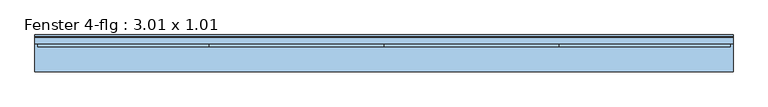
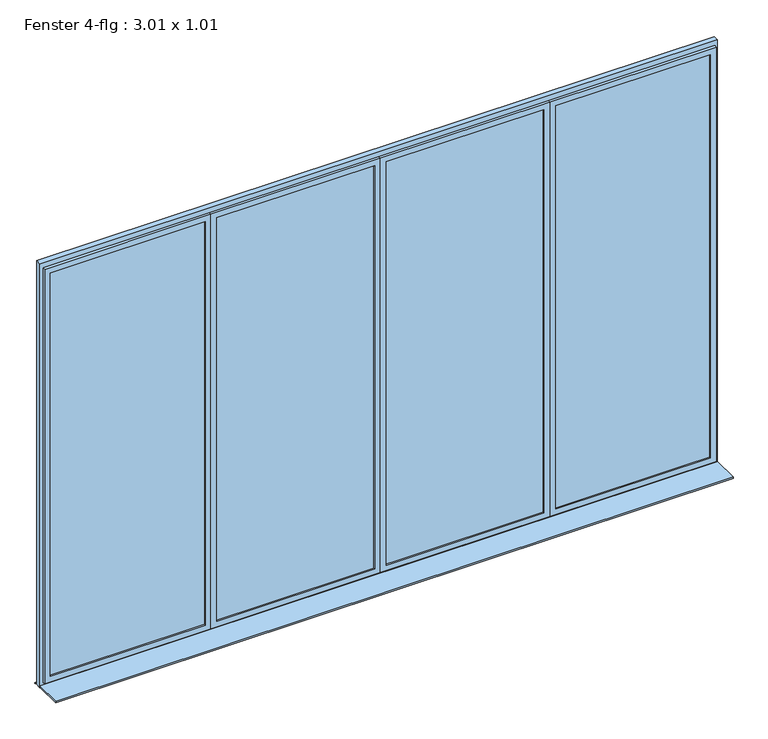
"""IFC4 building model written with IfcOpenShell, lengths in millimetres: window geometry, Fenster 4-flg : 3.01 x 1.01."""

import ifcopenshell
import ifcopenshell.guid

model = None  # the IFC model being written
_history = None  # IfcOwnerHistory: only IFC2X3 demands one
_inside = {}  # id of a spatial element -> (the spatial element, [elements in it])
_under = {}  # id of a project, library or spatial element -> (it, [spatial elements below it])
_declared = {}  # id of a project -> (the project, [libraries it declares])
_typed = {}  # id of a type object -> (the type object, [elements of that type])
_made_of = {}  # id of a material, layer set ... -> (it, [elements and type objects made of it])


def new_model(schema):
    """Start an empty IFC model of exactly this schema.

    Asked for "IFC4X3", IfcOpenShell would pick the latest addendum, in which some entities
    have other attributes; the version numbers below select the first issue.
    IFC2X3 requires an IfcOwnerHistory on every rooted entity: one is made here for all.
    """
    global model, _history
    if schema == "IFC4X3":
        model = ifcopenshell.file(schema_version=(4, 3, 0, 0))
    else:
        model = ifcopenshell.file(schema=schema)
    _inside.clear()
    _under.clear()
    _declared.clear()
    _typed.clear()
    _made_of.clear()
    _history = None
    if model.schema == "IFC2X3":
        org = make("IfcOrganization", Name="unknown")
        user = make(
            "IfcPersonAndOrganization",
            ThePerson=make("IfcPerson", FamilyName="unknown"),
            TheOrganization=org,
        )
        app = make(
            "IfcApplication",
            ApplicationDeveloper=org,
            Version="unknown",
            ApplicationFullName="unknown",
            ApplicationIdentifier="unknown",
        )
        _history = make(
            "IfcOwnerHistory",
            OwningUser=user,
            OwningApplication=app,
            ChangeAction="ADDED",
            CreationDate=0,
        )
    return model


def make(cls, **values):
    """One entity of the class cls with the attributes given. An attribute that is None is left unset."""
    return model.create_entity(
        cls, **{name: value for name, value in values.items() if value is not None}
    )


def rooted(cls, **values):
    """An entity with a GlobalId (a new one), such as an element, a storey or a relation."""
    return make(cls, GlobalId=ifcopenshell.guid.new(), OwnerHistory=_history, **values)


def si_unit(unit_type, name, prefix=None):
    """IfcSIUnit, for example si_unit("LENGTHUNIT", "METRE", prefix="MILLI")."""
    return make("IfcSIUnit", UnitType=unit_type, Prefix=prefix, Name=name)


def assignment(units):
    """IfcUnitAssignment: the units of a project."""
    return None if units is None else make("IfcUnitAssignment", Units=units)


def point(xyz):
    """IfcCartesianPoint."""
    return None if xyz is None else make("IfcCartesianPoint", Coordinates=xyz)


def direction(xyz):
    """IfcDirection."""
    return None if xyz is None else make("IfcDirection", DirectionRatios=xyz)


def frame(location, z_axis=None, x_axis=None):
    """IfcAxis2Placement3D, a coordinate frame: its origin and axes. An axis left out is left unset."""
    return make(
        "IfcAxis2Placement3D",
        Location=point(location),
        Axis=direction(z_axis),
        RefDirection=direction(x_axis),
    )


def origin():
    """The frame at (0, 0, 0) with its axes left unset."""
    return frame((0.0, 0.0, 0.0))


def place(relative_to, where):
    """IfcLocalPlacement: puts the frame where relative to a parent placement (None: the world)."""
    return make(
        "IfcLocalPlacement", PlacementRelTo=relative_to, RelativePlacement=where
    )


def context(
    kind, dimensions, precision=None, world=None, true_north=None, identifier=None
):
    """IfcGeometricRepresentationContext, for example the 3D "Model" context."""
    return make(
        "IfcGeometricRepresentationContext",
        ContextIdentifier=identifier,
        ContextType=kind,
        CoordinateSpaceDimension=dimensions,
        Precision=precision,
        WorldCoordinateSystem=world,
        TrueNorth=true_north,
    )


def project(units=None, contexts=None):
    """IfcProject with its units and contexts."""
    return rooted(
        "IfcProject",
        Name="project",
        RepresentationContexts=contexts,
        UnitsInContext=assignment(units),
    )


def spatial(cls, under=None, at=None, **own):
    """A site, building, storey or space (cls), placed at a placement, below another one or the project."""
    s = rooted(cls, ObjectPlacement=at, **own)
    if under is not None:
        _under.setdefault(under.id(), (under, []))[1].append(s)
    return s


def polyline(points):
    """IfcPolyline through the points."""
    return make("IfcPolyline", Points=[point(p) for p in points])


def outline(outer, holes=None, kind="AREA"):
    """IfcArbitraryClosedProfileDef: a profile drawn as a closed curve; with holes, ...WithVoids."""
    if holes is None:
        return make("IfcArbitraryClosedProfileDef", ProfileType=kind, OuterCurve=outer)
    return make(
        "IfcArbitraryProfileDefWithVoids",
        ProfileType=kind,
        OuterCurve=outer,
        InnerCurves=holes,
    )


def extrude(swept, where, along, depth):
    """IfcExtrudedAreaSolid: the profile swept, set in the frame where, extruded along a direction by depth."""
    return make(
        "IfcExtrudedAreaSolid",
        SweptArea=swept,
        Position=where,
        ExtrudedDirection=direction(along),
        Depth=depth,
    )


def faces_of(points, faces, orient=None, outer=None):
    """IfcFace entities. A face is a list of loops; a loop is a list of indices into points, from 0.

    orient and outer hold one flag for each loop. By default every Orientation is true, the
    first loop of a face is its IfcFaceOuterBound and the others are IfcFaceBound.
    """
    made = []
    for i, loops in enumerate(faces):
        bounds = []
        for j, loop in enumerate(loops):
            is_outer = j == 0 if outer is None else outer[i][j]
            bounds.append(
                make(
                    "IfcFaceOuterBound" if is_outer else "IfcFaceBound",
                    Bound=make("IfcPolyLoop", Polygon=[points[k] for k in loop]),
                    Orientation=True if orient is None else orient[i][j],
                )
            )
        made.append(make("IfcFace", Bounds=bounds))
    return made


def faceted_brep(points, faces, orient=None, outer=None, voids=None):
    """IfcFacetedBrep: a solid bounded by flat faces; with voids (closed shells), ...WithVoids."""
    shared = [point(p) for p in points]
    hull = make("IfcClosedShell", CfsFaces=faces_of(shared, faces, orient, outer))
    if voids is None:
        return make("IfcFacetedBrep", Outer=hull)
    return make(
        "IfcFacetedBrepWithVoids",
        Outer=hull,
        Voids=[
            make(cls, CfsFaces=faces_of(shared, fs, o, b)) for cls, fs, o, b in voids
        ],
    )


def shape(context_of_items, identifier, shape_type, items):
    """IfcShapeRepresentation: the items that make up one representation, for example the "Body"."""
    return make(
        "IfcShapeRepresentation",
        ContextOfItems=context_of_items,
        RepresentationIdentifier=identifier,
        RepresentationType=shape_type,
        Items=items,
    )


def source(mapping_origin, context_of_items, identifier, shape_type, items):
    """IfcRepresentationMap: a shape defined once, which mapped items show again and again."""
    return make(
        "IfcRepresentationMap",
        MappingOrigin=mapping_origin,
        MappedRepresentation=shape(context_of_items, identifier, shape_type, items),
    )


def transform(
    local_origin,
    x_axis=None,
    y_axis=None,
    z_axis=None,
    scale=None,
    scale2=None,
    scale3=None,
    uniform=True,
):
    """IfcCartesianTransformationOperator3D, or its non-uniform kind. x_axis, y_axis, z_axis: its Axis1, 2, 3."""
    if uniform:
        return make(
            "IfcCartesianTransformationOperator3D",
            Axis1=direction(x_axis),
            Axis2=direction(y_axis),
            LocalOrigin=point(local_origin),
            Scale=scale,
            Axis3=direction(z_axis),
        )
    return make(
        "IfcCartesianTransformationOperator3DnonUniform",
        Axis1=direction(x_axis),
        Axis2=direction(y_axis),
        LocalOrigin=point(local_origin),
        Scale=scale,
        Axis3=direction(z_axis),
        Scale2=scale2,
        Scale3=scale3,
    )


def mapped(mapping_source, mapping_target):
    """IfcMappedItem: shows the shape of a source again, moved by a transform."""
    return make(
        "IfcMappedItem", MappingSource=mapping_source, MappingTarget=mapping_target
    )


def made_of(thing, what):
    """Note that an element or type object is made of a material, layer set ...; save() writes the relation."""
    if what is not None:
        _made_of.setdefault(what.id(), (what, []))[1].append(thing)
    return thing


def element(
    cls,
    number,
    at=None,
    inside=None,
    cuts=None,
    type_object=None,
    material=None,
    context=None,
    identifier="Body",
    shape_type=None,
    held_by="IfcProductDefinitionShape",
    body=None,
    shapes=None,
    **own,
):
    """One element of the class cls, such as IfcWall. Its Tag is "e" and its number.

    at: its placement. inside: the storey or other place that contains it. cuts: it is an
    opening in that element (IfcRelVoidsElement). A single representation is given by context,
    identifier, shape_type and body (its items); several are given by shapes. held_by: the class
    of the entity that holds the representations. save() writes the other relations.
    """
    e = rooted(cls, Tag="e%d" % number, ObjectPlacement=at, **own)
    if body is not None:
        shapes = [shape(context, identifier, shape_type, body)]
    if shapes is not None:
        e.Representation = make(held_by, Representations=shapes)
    if inside is not None:
        _inside.setdefault(inside.id(), (inside, []))[1].append(e)
    if cuts is not None:
        rooted(
            "IfcRelVoidsElement", RelatingBuildingElement=cuts, RelatedOpeningElement=e
        )
    if type_object is not None:
        _typed.setdefault(type_object.id(), (type_object, []))[1].append(e)
    return made_of(e, material)


def aggregate(whole, parts):
    """IfcRelAggregates: a whole, such as a stair, and the parts it consists of."""
    return rooted("IfcRelAggregates", RelatingObject=whole, RelatedObjects=parts)


def save(model, path):
    """Write the relations noted so far, then the file.

    IfcRelAggregates (storeys below a building ...), IfcRelContainedInSpatialStructure (elements
    in a storey), IfcRelDefinesByType, IfcRelAssociatesMaterial and IfcRelDeclares: one each for
    every whole, place, type object, material and project.
    """
    for whole, parts in _under.values():
        aggregate(whole, parts)
    for where, things in _inside.values():
        rooted(
            "IfcRelContainedInSpatialStructure",
            RelatedElements=things,
            RelatingStructure=where,
        )
    for kind, things in _typed.values():
        rooted("IfcRelDefinesByType", RelatedObjects=things, RelatingType=kind)
    for what, things in _made_of.values():
        rooted("IfcRelAssociatesMaterial", RelatedObjects=things, RelatingMaterial=what)
    for by, libraries in _declared.values():
        rooted("IfcRelDeclares", RelatingContext=by, RelatedDefinitions=libraries)
    model.write(path)


def fenster_4_flg_3_01_x_1_01_20ed2dc3(model_context):
    return source(origin(), model_context, "Body", "SolidModel", [
        extrude(outline(polyline([(4150.75, 155.0), (4150.75, 95.0), (4090.75, 95.0), (4090.75, 155.0), (4150.75, 155.0)])), frame((0.0, 0.0, 1080.0), z_axis=(0.0, 0.0, 1.0), x_axis=(1.0, 0.0, 0.0)), (0.0, 0.0, 1.0), 4470.0),
        extrude(outline(polyline([(2400.5, 155.0), (2400.5, 95.0), (2340.5, 95.0), (2340.5, 155.0), (2400.5, 155.0)])), frame((0.0, 0.0, 1080.0), z_axis=(0.0, 0.0, 1.0), x_axis=(1.0, 0.0, 0.0)), (0.0, 0.0, 1.0), 4470.0),
        extrude(outline(polyline([(650.25, 155.0), (650.25, 95.0), (590.25, 95.0), (590.25, 155.0), (650.25, 155.0)])), frame((0.0, 0.0, 1080.0), z_axis=(0.0, 0.0, 1.0), x_axis=(1.0, 0.0, 0.0)), (0.0, 0.0, 1.0), 4470.0),
        extrude(outline(polyline([(5630.0, 5871.0), (5630.0, -1130.0), (1000.0, -1130.0), (1000.0, 5871.0), (5630.0, 5871.0)]), holes=[polyline([(5550.0, 5811.0), (1080.0, 5811.0), (1080.0, -1070.0), (5550.0, -1070.0), (5550.0, 5811.0)])]), frame((0.0, 95.0, 0.0), z_axis=(0.0, 1.0, 0.0), x_axis=(0.0, 0.0, 1.0)), (0.0, 0.0, 1.0), 60.0),
        faceted_brep([(4120.75, 95.0, 5580.0), (4120.75, 65.0, 5580.0), (4120.75, 65.0, 1050.0), (4120.75, 95.0, 1050.0), (2370.5, 65.0, 5580.0), (2370.5, 65.0, 1050.0), (4060.75, 65.0, 1110.0), (2430.5, 65.0, 1110.0), (2430.5, 65.0, 5520.0), (4060.75, 65.0, 5520.0), (2370.5, 95.0, 1050.0), (2370.5, 95.0, 5580.0), (4090.75, 95.0, 5550.0), (2400.5, 95.0, 5550.0), (2400.5, 95.0, 1080.0), (4090.75, 95.0, 1080.0), (4090.75, 125.0, 5550.0), (4090.75, 125.0, 1080.0), (2400.5, 125.0, 1080.0), (2400.5, 125.0, 5550.0), (4060.75, 125.0, 5520.0), (2430.5, 125.0, 5520.0), (2430.5, 125.0, 1110.0), (4060.75, 125.0, 1110.0)], [[[0, 1, 2, 3]], [[1, 4, 5, 2], [6, 7, 8, 9]], [[3, 2, 5, 10]], [[3, 10, 11, 0], [12, 13, 14, 15]], [[16, 12, 15, 17]], [[17, 15, 14, 18]], [[17, 18, 19, 16], [20, 21, 22, 23]], [[9, 20, 23, 6]], [[6, 23, 22, 7]], [[10, 5, 4, 11]], [[18, 14, 13, 19]], [[7, 22, 21, 8]], [[11, 4, 1, 0]], [[19, 13, 12, 16]], [[8, 21, 20, 9]]]),
        faceted_brep([(2370.5, 95.0, 5580.0), (2370.5, 65.0, 5580.0), (2370.5, 65.0, 1050.0), (2370.5, 95.0, 1050.0), (620.25, 65.0, 5580.0), (620.25, 65.0, 1050.0), (2310.5, 65.0, 1110.0), (680.25, 65.0, 1110.0), (680.25, 65.0, 5520.0), (2310.5, 65.0, 5520.0), (620.25, 95.0, 1050.0), (620.25, 95.0, 5580.0), (2340.5, 95.0, 5550.0), (650.25, 95.0, 5550.0), (650.25, 95.0, 1080.0), (2340.5, 95.0, 1080.0), (2340.5, 125.0, 5550.0), (2340.5, 125.0, 1080.0), (650.25, 125.0, 1080.0), (650.25, 125.0, 5550.0), (2310.5, 125.0, 5520.0), (680.25, 125.0, 5520.0), (680.25, 125.0, 1110.0), (2310.5, 125.0, 1110.0)], [[[0, 1, 2, 3]], [[1, 4, 5, 2], [6, 7, 8, 9]], [[3, 2, 5, 10]], [[3, 10, 11, 0], [12, 13, 14, 15]], [[16, 12, 15, 17]], [[17, 15, 14, 18]], [[17, 18, 19, 16], [20, 21, 22, 23]], [[9, 20, 23, 6]], [[6, 23, 22, 7]], [[10, 5, 4, 11]], [[18, 14, 13, 19]], [[7, 22, 21, 8]], [[11, 4, 1, 0]], [[19, 13, 12, 16]], [[8, 21, 20, 9]]]),
        faceted_brep([(620.25, 95.0, 5580.0), (620.25, 65.0, 5580.0), (620.25, 65.0, 1050.0), (620.25, 95.0, 1050.0), (-1100.0, 65.0, 5580.0), (-1100.0, 65.0, 1050.0), (560.25, 65.0, 1110.0), (-1040.0, 65.0, 1110.0), (-1040.0, 65.0, 5520.0), (560.25, 65.0, 5520.0), (-1100.0, 95.0, 1050.0), (-1100.0, 95.0, 5580.0), (590.25, 95.0, 5550.0), (-1070.0, 95.0, 5550.0), (-1070.0, 95.0, 1080.0), (590.25, 95.0, 1080.0), (590.25, 125.0, 5550.0), (590.25, 125.0, 1080.0), (-1070.0, 125.0, 1080.0), (-1070.0, 125.0, 5550.0), (560.25, 125.0, 5520.0), (-1040.0, 125.0, 5520.0), (-1040.0, 125.0, 1110.0), (560.25, 125.0, 1110.0)], [[[0, 1, 2, 3]], [[1, 4, 5, 2], [6, 7, 8, 9]], [[3, 2, 5, 10]], [[3, 10, 11, 0], [12, 13, 14, 15]], [[16, 12, 15, 17]], [[17, 15, 14, 18]], [[17, 18, 19, 16], [20, 21, 22, 23]], [[9, 20, 23, 6]], [[6, 23, 22, 7]], [[10, 5, 4, 11]], [[18, 14, 13, 19]], [[7, 22, 21, 8]], [[11, 4, 1, 0]], [[19, 13, 12, 16]], [[8, 21, 20, 9]]]),
        faceted_brep([(5841.0, 95.0, 5580.0), (5841.0, 65.0, 5580.0), (5841.0, 65.0, 1050.0), (5841.0, 95.0, 1050.0), (4120.75, 65.0, 5580.0), (4120.75, 65.0, 1050.0), (5781.0, 65.0, 1110.0), (4180.75, 65.0, 1110.0), (4180.75, 65.0, 5520.0), (5781.0, 65.0, 5520.0), (4120.75, 95.0, 1050.0), (4120.75, 95.0, 5580.0), (5811.0, 95.0, 5550.0), (4150.75, 95.0, 5550.0), (4150.75, 95.0, 1080.0), (5811.0, 95.0, 1080.0), (5811.0, 125.0, 5550.0), (5811.0, 125.0, 1080.0), (4150.75, 125.0, 1080.0), (4150.75, 125.0, 5550.0), (5781.0, 125.0, 5520.0), (4180.75, 125.0, 5520.0), (4180.75, 125.0, 1110.0), (5781.0, 125.0, 1110.0)], [[[0, 1, 2, 3]], [[1, 4, 5, 2], [6, 7, 8, 9]], [[3, 2, 5, 10]], [[3, 10, 11, 0], [12, 13, 14, 15]], [[16, 12, 15, 17]], [[17, 15, 14, 18]], [[17, 18, 19, 16], [20, 21, 22, 23]], [[9, 20, 23, 6]], [[6, 23, 22, 7]], [[10, 5, 4, 11]], [[18, 14, 13, 19]], [[7, 22, 21, 8]], [[11, 4, 1, 0]], [[19, 13, 12, 16]], [[8, 21, 20, 9]]]),
        extrude(outline(polyline([(165.0221543, 1020.0), (185.0, 1000.0), (185.0, 990.0), (183.0, 990.0), (183.0, 998.3604634), (164.8240723, 1018.0), (155.0, 1018.0), (155.0, 1020.0), (165.0221543, 1020.0)])), frame((-1130.0, 0.0, 0.0), z_axis=(1.0, 0.0, 0.0), x_axis=(0.0, 1.0, 0.0)), (0.0, 0.0, 1.0), 7001.0),
        extrude(outline(polyline([(-1130.0, -185.0), (-1130.0, 95.0), (5871.0, 95.0), (5871.0, -185.0), (-1130.0, -185.0)])), frame((0.0, 0.0, 1005.0), z_axis=(0.0, 0.0, 1.0), x_axis=(1.0, 0.0, 0.0)), (0.0, 0.0, 1.0), 15.0),
        extrude(outline(polyline([(560.25, 80.0), (-1040.0, 80.0), (-1040.0, 110.0), (560.25, 110.0), (560.25, 80.0)])), frame((0.0, 0.0, 1110.0), z_axis=(0.0, 0.0, 1.0), x_axis=(1.0, 0.0, 0.0)), (0.0, 0.0, 1.0), 4410.0),
        extrude(outline(polyline([(2310.5, 80.0), (680.25, 80.0), (680.25, 110.0), (2310.5, 110.0), (2310.5, 80.0)])), frame((0.0, 0.0, 1110.0), z_axis=(0.0, 0.0, 1.0), x_axis=(1.0, 0.0, 0.0)), (0.0, 0.0, 1.0), 4410.0),
        extrude(outline(polyline([(4060.75, 80.0), (2430.5, 80.0), (2430.5, 110.0), (4060.75, 110.0), (4060.75, 80.0)])), frame((0.0, 0.0, 1110.0), z_axis=(0.0, 0.0, 1.0), x_axis=(1.0, 0.0, 0.0)), (0.0, 0.0, 1.0), 4410.0),
        extrude(outline(polyline([(5781.0, 80.0), (4180.75, 80.0), (4180.75, 110.0), (5781.0, 110.0), (5781.0, 80.0)])), frame((0.0, 0.0, 1110.0), z_axis=(0.0, 0.0, 1.0), x_axis=(1.0, 0.0, 0.0)), (0.0, 0.0, 1.0), 4410.0),
    ])


if __name__ == "__main__":
    model = new_model("IFC4")
    model_context = context("Model", 3, world=origin())
    ifc_project = project(units=[si_unit("LENGTHUNIT", "METRE", prefix="MILLI")], contexts=[model_context])
    site = spatial("IfcSite", under=ifc_project)
    building = spatial("IfcBuilding", under=site)
    placement = place(None, origin())
    fenster_4_flg_3_01_x_1_01_shape = fenster_4_flg_3_01_x_1_01_20ed2dc3(model_context)
    element("IfcWindow", 1, ObjectType="Fenster 4-flg : 3.01 x 1.01", at=placement, inside=building, context=model_context, shape_type="MappedRepresentation", body=[
        mapped(fenster_4_flg_3_01_x_1_01_shape, transform((0.0, 0.0, 0.0), x_axis=(1.0, 0.0, 0.0), y_axis=(0.0, 1.0, 0.0), z_axis=(0.0, 0.0, 1.0))),
    ])
    save(model, "model.ifc")

# Revit data of these elements
# Project information
#   Projektausgabedatum = "Projekt Datum"
#   Projektstatus = "Projektstatus"
#   Kundenname = "Bauherr"
#   Projektadresse = "Projektadresse"
#   Projektname = "Projektname"
#   Projektnummer = "Projektnummer"
#   Verfasser Firma 1 = "Firma 1"
#   Verfasser Firma 2 = "Firma 2"
#   Verfasser PLZ Ort = "PLZ Ort"
#   Verfasser Strasse = "Strasse"
#   Verfasser Telefon = "Telefon"
#   Verfasser Telefax = "Telefax"
#   Verfasser eMail = "E-Mail"
# Type "Fenster 4-flg : 3.01 x 1.01"
#   Type Mark = "51"
#   Operation = "UserDefined"
#   Keynote = "16.05.01"
#   Visual Light Transmittance = 0.9
#   Solar Heat Gain Coefficient = 0.78
#   Rough Height = 4.630 m
#   Rough Width = 7.001 m
#   Heat Transfer Coefficient (U) = 3.6886 W/(m²·K)
#   Rahmentiefe = 0.060 m
#   Breite unterer Rahmen = 0.080 m
#   Breite oberer  Rahmen = 0.080 m
#   Rahmenbreite = 0.060 m
#   Height = 4.630 m
#   Tiefe Flügel = 0.060 m
#   Flügelbreite = 0.060 m
#   Einbautiefe (von außen) [instance default] = 0.080 m
#   Width = 7.001 m
#   Bild = Metall - Aluminium
#   Glas = Fenster - Glas
#   Fensterflügel = Metall - Aluminium
#   Innere Fensterbank = Metall - Aluminium
#   Äußere Fensterbank = Metall - Aluminium
#   Construction Type Id = ""
#   Wall Closure = (empty or 0)
#   Analytic Construction = (empty or 0)
# Element 1 (IfcWindow, "Fenster 4-flg : 3.01 x 1.01")
#   Einbautiefe (von außen) = 0.000 m
#   Materials on its faces: "Metall - Aluminium", "Fenster - Glas"
# Materials
#   "Metall - Aluminium": class "Metall", colour RGB 247 247 247, transparency 0, Description = "Aluminium 6061", Cost = 0
#   "Fenster - Glas": class "Glas", colour RGB 128 128 255, transparency 0.75, Cost = 0
